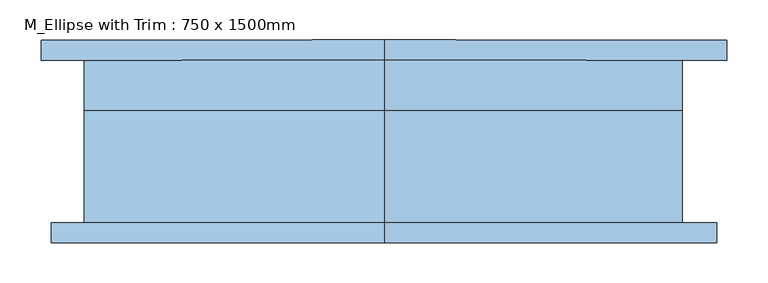
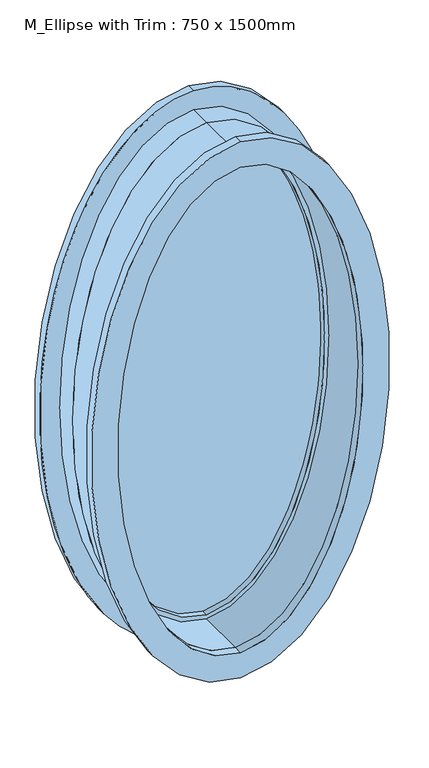
"""IFC4 building model written with IfcOpenShell, lengths in millimetres: window geometry, M_Ellipse with Trim : 750 x 1500mm."""

from ifc_helpers import new_model, si_unit, point, frame, origin, place, context, project, spatial, ellipse_curve, trimmed, source, transform, mapped, element, save
from ifc_brep_helpers import plane_surface, extruded_surface, advanced_brep


def m_ellipse_with_trim_750_x_1500mm_90dfdbfc(model_context):
    return source(origin(), model_context, "Body", "AdvancedBrep", [
        advanced_brep(
        [(0.0, -101.6, 2415.0), (0.0, -101.6, 915.0), (0.0, -101.6, 2383.25), (0.0, -101.6, 946.75), (0.0, 38.1, 2415.0), (0.0, 38.1, 915.0), (0.0, 38.1, 2383.25), (0.0, 38.1, 946.75)],
        [
            (0, 1, ellipse_curve(frame((0.0, -101.6, 1665.0), z_axis=(0.0, -1.0, 0.0), x_axis=(0.0, 0.0, -1.0)), 750.0, 375.0)),
            (1, 0, ellipse_curve(frame((0.0, -101.6, 1665.0), z_axis=(0.0, -1.0, 0.0), x_axis=(0.0, 0.0, -1.0)), 750.0, 375.0)),
            (2, 3, ellipse_curve(frame((0.0, -101.6, 1665.0), z_axis=(0.0, 1.0, 0.0), x_axis=(0.0, 0.0, -1.0)), 718.25, 343.25)),
            (3, 2, ellipse_curve(frame((0.0, -101.6, 1665.0), z_axis=(0.0, 1.0, 0.0), x_axis=(0.0, 0.0, -1.0)), 718.25, 343.25)),
            (0, 4),
            (4, 5, ellipse_curve(frame((0.0, 38.1, 1665.0), z_axis=(0.0, -1.0, 0.0), x_axis=(0.0, 0.0, -1.0)), 750.0, 375.0)),
            (5, 1),
            (5, 4, ellipse_curve(frame((0.0, 38.1, 1665.0), z_axis=(0.0, -1.0, 0.0), x_axis=(0.0, 0.0, -1.0)), 750.0, 375.0)),
            (2, 6),
            (6, 7, ellipse_curve(frame((0.0, 38.1, 1665.0), z_axis=(0.0, 1.0, 0.0), x_axis=(0.0, 0.0, -1.0)), 718.25, 343.25)),
            (7, 3),
            (7, 6, ellipse_curve(frame((0.0, 38.1, 1665.0), z_axis=(0.0, 1.0, 0.0), x_axis=(0.0, 0.0, -1.0)), 718.25, 343.25)),
        ],
        [
            plane_surface(frame((0.0, -101.6, 915.0), z_axis=(0.0, -1.0, 0.0), x_axis=(1.0, 0.0, 0.0))),
            extruded_surface(trimmed(ellipse_curve(frame((0.0, 177.8, 1665.0), z_axis=(0.0, -1.0, 0.0), x_axis=(0.0, 0.0, -1.0)), 750.0, 375.0), [point((0.0, 177.8, 2415.0))], [point((0.0, 177.8, 915.0))], True, "CARTESIAN"), (0.0, -139.70000000000002, 0.0), 139.70000000000002),
            extruded_surface(trimmed(ellipse_curve(frame((0.0, 177.8, 1665.0), z_axis=(0.0, -1.0, 0.0), x_axis=(0.0, 0.0, -1.0)), 750.0, 375.0), [point((0.0, 177.8, 915.0))], [point((0.0, 177.8, 2415.0))], True, "CARTESIAN"), (0.0, -139.70000000000002, 0.0), 139.70000000000002),
            extruded_surface(trimmed(ellipse_curve(frame((0.0, 38.1, 1665.0), z_axis=(0.0, 1.0, 0.0), x_axis=(0.0, 0.0, -1.0)), 718.25, 343.25), [point((0.0, 38.1, 2383.25))], [point((0.0, 38.1, 946.75))], True, "CARTESIAN"), (0.0, -139.7, 0.0), 139.7),
            extruded_surface(trimmed(ellipse_curve(frame((0.0, 38.1, 1665.0), z_axis=(0.0, 1.0, 0.0), x_axis=(0.0, 0.0, -1.0)), 718.25, 343.25), [point((0.0, 38.1, 946.75))], [point((0.0, 38.1, 2383.25))], True, "CARTESIAN"), (0.0, -139.7, 0.0), 139.7),
            plane_surface(frame((0.0, 38.1, 915.0), z_axis=(0.0, 1.0, 0.0), x_axis=(-1.0, 0.0, 0.0))),
        ],
        [
            (0, [[1, 2], [3, 4]]),
            (1, [[-1, 5, 6, 7]]),
            (2, [[-2, -7, 8, -5]]),
            (3, [[-3, 9, 10, 11]]),
            (4, [[-4, -11, 12, -9]]),
            (5, [[-8, -6], [-12, -10]]),
        ],
    ),
        advanced_brep(
        [(0.0, 55.3459129, 2370.55), (0.0, 55.3459129, 959.45), (0.0, 64.8706843, 2370.55), (0.0, 64.8706843, 959.45)],
        [
            (0, 1, ellipse_curve(frame((0.0, 55.3459129, 1665.0), z_axis=(0.0, -1.0, 0.0), x_axis=(0.0, 0.0, -1.0)), 705.55, 330.55)),
            (1, 0, ellipse_curve(frame((0.0, 55.3459129, 1665.0), z_axis=(0.0, -1.0, 0.0), x_axis=(0.0, 0.0, -1.0)), 705.55, 330.55)),
            (0, 2),
            (2, 3, ellipse_curve(frame((0.0, 64.8706843, 1665.0), z_axis=(0.0, -1.0, 0.0), x_axis=(0.0, 0.0, -1.0)), 705.55, 330.55)),
            (3, 1),
            (3, 2, ellipse_curve(frame((0.0, 64.8706843, 1665.0), z_axis=(0.0, -1.0, 0.0), x_axis=(0.0, 0.0, -1.0)), 705.55, 330.55)),
        ],
        [
            plane_surface(frame((0.0, 55.3459129, 959.45), z_axis=(0.0, -1.0, 0.0), x_axis=(1.0, 0.0, 0.0))),
            extruded_surface(trimmed(ellipse_curve(frame((0.0, 74.3954558, 1665.0), z_axis=(0.0, -1.0, 0.0), x_axis=(0.0, 0.0, -1.0)), 705.55, 330.55), [point((0.0, 74.3954558, 2370.55))], [point((0.0, 74.3954558, 959.45))], True, "CARTESIAN"), (0.0, -9.5247715, 0.0), 9.5247715),
            extruded_surface(trimmed(ellipse_curve(frame((0.0, 74.3954558, 1665.0), z_axis=(0.0, -1.0, 0.0), x_axis=(0.0, 0.0, -1.0)), 705.55, 330.55), [point((0.0, 74.3954558, 959.45))], [point((0.0, 74.3954558, 2370.55))], True, "CARTESIAN"), (0.0, -9.5247715, 0.0), 9.5247715),
            plane_surface(frame((0.0, 64.8706843, 959.45), z_axis=(0.0, 1.0, 0.0), x_axis=(-1.0, 0.0, 0.0))),
        ],
        [
            (0, [[1, 2]]),
            (1, [[-1, 3, 4, 5]]),
            (2, [[-2, -5, 6, -3]]),
            (3, [[-6, -4]]),
        ],
    ),
        advanced_brep(
        [(0.0, 38.1, 2395.95), (0.0, 38.1, 934.05), (0.0, 38.1, 2370.55), (0.0, 38.1, 959.45), (0.0, 82.55, 2395.95), (0.0, 82.55, 934.05), (0.0, 82.55, 2370.55), (0.0, 82.55, 959.45)],
        [
            (0, 1, ellipse_curve(frame((0.0, 38.1, 1665.0), z_axis=(0.0, -1.0, 0.0), x_axis=(0.0, 0.0, -1.0)), 730.95, 355.95)),
            (1, 0, ellipse_curve(frame((0.0, 38.1, 1665.0), z_axis=(0.0, -1.0, 0.0), x_axis=(0.0, 0.0, -1.0)), 730.95, 355.95)),
            (2, 3, ellipse_curve(frame((0.0, 38.1, 1665.0), z_axis=(0.0, 1.0, 0.0), x_axis=(0.0, 0.0, -1.0)), 705.55, 330.55)),
            (3, 2, ellipse_curve(frame((0.0, 38.1, 1665.0), z_axis=(0.0, 1.0, 0.0), x_axis=(0.0, 0.0, -1.0)), 705.55, 330.55)),
            (0, 4),
            (4, 5, ellipse_curve(frame((0.0, 82.55, 1665.0), z_axis=(0.0, -1.0, 0.0), x_axis=(0.0, 0.0, -1.0)), 730.95, 355.95)),
            (5, 1),
            (5, 4, ellipse_curve(frame((0.0, 82.55, 1665.0), z_axis=(0.0, -1.0, 0.0), x_axis=(0.0, 0.0, -1.0)), 730.95, 355.95)),
            (2, 6),
            (6, 7, ellipse_curve(frame((0.0, 82.55, 1665.0), z_axis=(0.0, 1.0, 0.0), x_axis=(0.0, 0.0, -1.0)), 705.55, 330.55)),
            (7, 3),
            (7, 6, ellipse_curve(frame((0.0, 82.55, 1665.0), z_axis=(0.0, 1.0, 0.0), x_axis=(0.0, 0.0, -1.0)), 705.55, 330.55)),
        ],
        [
            plane_surface(frame((0.0, 38.1, 934.05), z_axis=(0.0, -1.0, 0.0), x_axis=(1.0, 0.0, 0.0))),
            extruded_surface(trimmed(ellipse_curve(frame((0.0, 127.0, 1665.0), z_axis=(0.0, -1.0, 0.0), x_axis=(0.0, 0.0, -1.0)), 730.95, 355.95), [point((0.0, 127.0, 2395.95))], [point((0.0, 127.0, 934.05))], True, "CARTESIAN"), (0.0, -44.45, 0.0), 44.45),
            extruded_surface(trimmed(ellipse_curve(frame((0.0, 127.0, 1665.0), z_axis=(0.0, -1.0, 0.0), x_axis=(0.0, 0.0, -1.0)), 730.95, 355.95), [point((0.0, 127.0, 934.05))], [point((0.0, 127.0, 2395.95))], True, "CARTESIAN"), (0.0, -44.45, 0.0), 44.45),
            extruded_surface(trimmed(ellipse_curve(frame((0.0, 146.05, 1665.0), z_axis=(0.0, 1.0, 0.0), x_axis=(0.0, 0.0, -1.0)), 705.55, 330.55), [point((0.0, 146.05, 2370.55))], [point((0.0, 146.05, 959.45))], True, "CARTESIAN"), (0.0, -44.45000000000002, 0.0), 44.45000000000002),
            extruded_surface(trimmed(ellipse_curve(frame((0.0, 146.05, 1665.0), z_axis=(0.0, 1.0, 0.0), x_axis=(0.0, 0.0, -1.0)), 705.55, 330.55), [point((0.0, 146.05, 959.45))], [point((0.0, 146.05, 2370.55))], True, "CARTESIAN"), (0.0, -44.45000000000002, 0.0), 44.45000000000002),
            plane_surface(frame((0.0, 82.55, 934.05), z_axis=(0.0, 1.0, 0.0), x_axis=(-1.0, 0.0, 0.0))),
        ],
        [
            (0, [[1, 2], [3, 4]]),
            (1, [[-1, 5, 6, 7]]),
            (2, [[-2, -7, 8, -5]]),
            (3, [[-3, 9, 10, 11]]),
            (4, [[-4, -11, 12, -9]]),
            (5, [[-8, -6], [-12, -10]]),
        ],
    ),
        advanced_brep(
        [(0.0, 38.1, 2415.0), (0.0, 38.1, 915.0), (0.0, 38.1, 2395.95), (0.0, 38.1, 934.05), (0.0, 101.6, 2415.0), (0.0, 101.6, 915.0), (0.0, 101.6, 2395.95), (0.0, 101.6, 934.05)],
        [
            (0, 1, ellipse_curve(frame((0.0, 38.1, 1665.0), z_axis=(0.0, -1.0, 0.0), x_axis=(0.0, 0.0, -1.0)), 750.0, 375.0)),
            (1, 0, ellipse_curve(frame((0.0, 38.1, 1665.0), z_axis=(0.0, -1.0, 0.0), x_axis=(0.0, 0.0, -1.0)), 750.0, 375.0)),
            (2, 3, ellipse_curve(frame((0.0, 38.1, 1665.0), z_axis=(0.0, 1.0, 0.0), x_axis=(0.0, 0.0, -1.0)), 730.95, 355.95)),
            (3, 2, ellipse_curve(frame((0.0, 38.1, 1665.0), z_axis=(0.0, 1.0, 0.0), x_axis=(0.0, 0.0, -1.0)), 730.95, 355.95)),
            (0, 4),
            (4, 5, ellipse_curve(frame((0.0, 101.6, 1665.0), z_axis=(0.0, -1.0, 0.0), x_axis=(0.0, 0.0, -1.0)), 750.0, 375.0)),
            (5, 1),
            (5, 4, ellipse_curve(frame((0.0, 101.6, 1665.0), z_axis=(0.0, -1.0, 0.0), x_axis=(0.0, 0.0, -1.0)), 750.0, 375.0)),
            (2, 6),
            (6, 7, ellipse_curve(frame((0.0, 101.6, 1665.0), z_axis=(0.0, 1.0, 0.0), x_axis=(0.0, 0.0, -1.0)), 730.95, 355.95)),
            (7, 3),
            (7, 6, ellipse_curve(frame((0.0, 101.6, 1665.0), z_axis=(0.0, 1.0, 0.0), x_axis=(0.0, 0.0, -1.0)), 730.95, 355.95)),
        ],
        [
            plane_surface(frame((0.0, 38.1, 915.0), z_axis=(0.0, -1.0, 0.0), x_axis=(1.0, 0.0, 0.0))),
            extruded_surface(trimmed(ellipse_curve(frame((0.0, 165.1, 1665.0), z_axis=(0.0, -1.0, 0.0), x_axis=(0.0, 0.0, -1.0)), 750.0, 375.0), [point((0.0, 165.1, 2415.0))], [point((0.0, 165.1, 915.0))], True, "CARTESIAN"), (0.0, -63.5, 0.0), 63.5),
            extruded_surface(trimmed(ellipse_curve(frame((0.0, 165.1, 1665.0), z_axis=(0.0, -1.0, 0.0), x_axis=(0.0, 0.0, -1.0)), 750.0, 375.0), [point((0.0, 165.1, 915.0))], [point((0.0, 165.1, 2415.0))], True, "CARTESIAN"), (0.0, -63.5, 0.0), 63.5),
            extruded_surface(trimmed(ellipse_curve(frame((0.0, 165.1, 1665.0), z_axis=(0.0, 1.0, 0.0), x_axis=(0.0, 0.0, -1.0)), 730.95, 355.95), [point((0.0, 165.1, 2395.95))], [point((0.0, 165.1, 934.05))], True, "CARTESIAN"), (0.0, -63.5, 0.0), 63.5),
            extruded_surface(trimmed(ellipse_curve(frame((0.0, 165.1, 1665.0), z_axis=(0.0, 1.0, 0.0), x_axis=(0.0, 0.0, -1.0)), 730.95, 355.95), [point((0.0, 165.1, 934.05))], [point((0.0, 165.1, 2395.95))], True, "CARTESIAN"), (0.0, -63.5, 0.0), 63.5),
            plane_surface(frame((0.0, 101.6, 915.0), z_axis=(0.0, 1.0, 0.0), x_axis=(-1.0, 0.0, 0.0))),
        ],
        [
            (0, [[1, 2], [3, 4]]),
            (1, [[-1, 5, 6, 7]]),
            (2, [[-2, -7, 8, -5]]),
            (3, [[-3, 9, 10, 11]]),
            (4, [[-4, -11, 12, -9]]),
            (5, [[-8, -6], [-12, -10]]),
        ],
    ),
        advanced_brep(
        [(0.0, -126.6, 2458.25), (0.0, -126.6, 871.75), (0.0, -126.6, 2383.25), (0.0, -126.6, 946.75), (0.0, -101.6, 2458.25), (0.0, -101.6, 871.75), (0.0, -101.6, 2383.25), (0.0, -101.6, 946.75)],
        [
            (0, 1, ellipse_curve(frame((0.0, -126.6, 1665.0), z_axis=(0.0, -1.0, 0.0), x_axis=(0.0, 0.0, -1.0)), 793.25, 418.25)),
            (1, 0, ellipse_curve(frame((0.0, -126.6, 1665.0), z_axis=(0.0, -1.0, 0.0), x_axis=(0.0, 0.0, -1.0)), 793.25, 418.25)),
            (2, 3, ellipse_curve(frame((0.0, -126.6, 1665.0), z_axis=(0.0, 1.0, 0.0), x_axis=(0.0, 0.0, -1.0)), 718.25, 343.25)),
            (3, 2, ellipse_curve(frame((0.0, -126.6, 1665.0), z_axis=(0.0, 1.0, 0.0), x_axis=(0.0, 0.0, -1.0)), 718.25, 343.25)),
            (4, 5, ellipse_curve(frame((0.0, -101.6, 1665.0), z_axis=(0.0, 1.0, 0.0), x_axis=(0.0, 0.0, -1.0)), 793.25, 418.25)),
            (5, 4, ellipse_curve(frame((0.0, -101.6, 1665.0), z_axis=(0.0, 1.0, 0.0), x_axis=(0.0, 0.0, -1.0)), 793.25, 418.25)),
            (6, 7, ellipse_curve(frame((0.0, -101.6, 1665.0), z_axis=(0.0, -1.0, 0.0), x_axis=(0.0, 0.0, -1.0)), 718.25, 343.25)),
            (7, 6, ellipse_curve(frame((0.0, -101.6, 1665.0), z_axis=(0.0, -1.0, 0.0), x_axis=(0.0, 0.0, -1.0)), 718.25, 343.25)),
            (2, 6),
            (7, 3),
            (0, 4),
            (5, 1),
        ],
        [
            plane_surface(frame((0.0, -126.6, 946.75), z_axis=(0.0, -1.0, 0.0), x_axis=(-1.0, 0.0, 0.0))),
            plane_surface(frame((0.0, -101.6, 946.75), z_axis=(0.0, 1.0, 0.0), x_axis=(1.0, 0.0, 0.0))),
            extruded_surface(trimmed(ellipse_curve(frame((0.0, -76.6, 1665.0), z_axis=(0.0, 1.0, 0.0), x_axis=(0.0, 0.0, -1.0)), 718.25, 343.25), [point((0.0, -76.6, 2383.25))], [point((0.0, -76.6, 946.75))], True, "CARTESIAN"), (0.0, -25.0, 0.0), 25.0),
            extruded_surface(trimmed(ellipse_curve(frame((0.0, -76.6, 1665.0), z_axis=(0.0, 1.0, 0.0), x_axis=(0.0, 0.0, -1.0)), 718.25, 343.25), [point((0.0, -76.6, 946.75))], [point((0.0, -76.6, 2383.25))], True, "CARTESIAN"), (0.0, -25.0, 0.0), 25.0),
            extruded_surface(trimmed(ellipse_curve(frame((0.0, -76.6, 1665.0), z_axis=(0.0, -1.0, 0.0), x_axis=(0.0, 0.0, -1.0)), 793.25, 418.25), [point((0.0, -76.6, 2458.25))], [point((0.0, -76.6, 871.75))], True, "CARTESIAN"), (0.0, -25.0, 0.0), 25.0),
            extruded_surface(trimmed(ellipse_curve(frame((0.0, -76.6, 1665.0), z_axis=(0.0, -1.0, 0.0), x_axis=(0.0, 0.0, -1.0)), 793.25, 418.25), [point((0.0, -76.6, 871.75))], [point((0.0, -76.6, 2458.25))], True, "CARTESIAN"), (0.0, -25.0, 0.0), 25.0),
        ],
        [
            (0, [[1, 2], [3, 4]]),
            (1, [[5, 6], [7, 8]]),
            (2, [[-3, 9, -8, 10]]),
            (3, [[-4, -10, -7, -9]]),
            (4, [[-1, 11, -6, 12]]),
            (5, [[-2, -12, -5, -11]]),
        ],
    ),
        advanced_brep(
        [(0.0, 101.6, 2470.95), (0.0, 101.6, 859.05), (0.0, 101.6, 2395.95), (0.0, 101.6, 934.05), (0.0, 126.6, 2470.95), (0.0, 126.6, 859.05), (0.0, 126.6, 2395.95), (0.0, 126.6, 934.05)],
        [
            (0, 1, ellipse_curve(frame((0.0, 101.6, 1665.0), z_axis=(0.0, -1.0, 0.0), x_axis=(0.0, 0.0, -1.0)), 805.95, 430.95)),
            (1, 0, ellipse_curve(frame((0.0, 101.6, 1665.0), z_axis=(0.0, -1.0, 0.0), x_axis=(0.0, 0.0, -1.0)), 805.95, 430.95)),
            (2, 3, ellipse_curve(frame((0.0, 101.6, 1665.0), z_axis=(0.0, 1.0, 0.0), x_axis=(0.0, 0.0, -1.0)), 730.95, 355.95)),
            (3, 2, ellipse_curve(frame((0.0, 101.6, 1665.0), z_axis=(0.0, 1.0, 0.0), x_axis=(0.0, 0.0, -1.0)), 730.95, 355.95)),
            (4, 5, ellipse_curve(frame((0.0, 126.6, 1665.0), z_axis=(0.0, 1.0, 0.0), x_axis=(0.0, 0.0, -1.0)), 805.95, 430.95)),
            (5, 4, ellipse_curve(frame((0.0, 126.6, 1665.0), z_axis=(0.0, 1.0, 0.0), x_axis=(0.0, 0.0, -1.0)), 805.95, 430.95)),
            (6, 7, ellipse_curve(frame((0.0, 126.6, 1665.0), z_axis=(0.0, -1.0, 0.0), x_axis=(0.0, 0.0, -1.0)), 730.95, 355.95)),
            (7, 6, ellipse_curve(frame((0.0, 126.6, 1665.0), z_axis=(0.0, -1.0, 0.0), x_axis=(0.0, 0.0, -1.0)), 730.95, 355.95)),
            (2, 6),
            (7, 3),
            (0, 4),
            (5, 1),
        ],
        [
            plane_surface(frame((0.0, 101.6, 934.05), z_axis=(0.0, -1.0, 0.0), x_axis=(-1.0, 0.0, 0.0))),
            plane_surface(frame((0.0, 126.6, 934.05), z_axis=(0.0, 1.0, 0.0), x_axis=(1.0, 0.0, 0.0))),
            extruded_surface(trimmed(ellipse_curve(frame((0.0, 151.6, 1665.0), z_axis=(0.0, 1.0, 0.0), x_axis=(0.0, 0.0, -1.0)), 730.95, 355.95), [point((0.0, 151.6, 2395.95))], [point((0.0, 151.6, 934.05))], True, "CARTESIAN"), (0.0, -25.0, 0.0), 25.0),
            extruded_surface(trimmed(ellipse_curve(frame((0.0, 151.6, 1665.0), z_axis=(0.0, 1.0, 0.0), x_axis=(0.0, 0.0, -1.0)), 730.95, 355.95), [point((0.0, 151.6, 934.05))], [point((0.0, 151.6, 2395.95))], True, "CARTESIAN"), (0.0, -25.0, 0.0), 25.0),
            extruded_surface(trimmed(ellipse_curve(frame((0.0, 126.6, 1665.0), z_axis=(0.0, -1.0, 0.0), x_axis=(0.0, 0.0, -1.0)), 805.95, 430.95), [point((0.0, 126.6, 2470.95))], [point((0.0, 126.6, 859.05))], True, "CARTESIAN"), (0.0, -25.0, 0.0), 25.0),
            extruded_surface(trimmed(ellipse_curve(frame((0.0, 126.6, 1665.0), z_axis=(0.0, -1.0, 0.0), x_axis=(0.0, 0.0, -1.0)), 805.95, 430.95), [point((0.0, 126.6, 859.05))], [point((0.0, 126.6, 2470.95))], True, "CARTESIAN"), (0.0, -25.0, 0.0), 25.0),
        ],
        [
            (0, [[1, 2], [3, 4]]),
            (1, [[5, 6], [7, 8]]),
            (2, [[-3, 9, -8, 10]]),
            (3, [[-4, -10, -7, -9]]),
            (4, [[-1, 11, -6, 12]]),
            (5, [[-2, -12, -5, -11]]),
        ],
    ),
    ])


if __name__ == "__main__":
    model = new_model("IFC4")
    model_context = context("Model", 3, world=origin())
    ifc_project = project(units=[si_unit("LENGTHUNIT", "METRE", prefix="MILLI")], contexts=[model_context])
    site = spatial("IfcSite", under=ifc_project)
    building = spatial("IfcBuilding", under=site)
    placement = place(None, origin())
    m_ellipse_with_trim_750_x_1500mm_shape = m_ellipse_with_trim_750_x_1500mm_90dfdbfc(model_context)
    element("IfcWindow", 1, ObjectType="M_Ellipse with Trim : 750 x 1500mm", at=placement, inside=building, context=model_context, shape_type="MappedRepresentation", body=[
        mapped(m_ellipse_with_trim_750_x_1500mm_shape, transform((0.0, 0.0, 0.0), x_axis=(1.0, 0.0, 0.0), y_axis=(0.0, 1.0, 0.0), z_axis=(0.0, 0.0, 1.0))),
    ])
    save(model, "model.ifc")

# Revit data of these elements
# Type "M_Ellipse with Trim : 750 x 1500mm"
#   Type Mark = "20"
#   Construction Type Id = "GSP4R"
#   Analytic Construction = "1/8 in Pilkington single glazing"
#   Visual Light Transmittance = 0.9
#   Thermal Resistance (R) = 0.1491 (m²·K)/W
#   Solar Heat Gain Coefficient = 0.86
#   Height = 4' - 11.05512"
#   Heat Transfer Coefficient (U) = 6.7069 W/(m²·K)
#   Half Width = 1' - 2.76378"
#   Half Height = 2' - 5.52756"
#   Default Sill Height = 3' - 0.02362"
#   Trim Projection = 0' - 0.98425"
#   Trim Width = 0' - 2.95276"
#   Width = 2' - 5.52756"
#   Trim Material = none
#   Sash Material = none
#   Wall Closure = (empty or 0)
# Element 1 (IfcWindow, "M_Ellipse with Trim : 750 x 1500mm")
#   Materials on its faces: "Glass"
# Materials
#   "Glass": class "Glass", colour RGB 0 128 192, transparency 0.75, Description = "Soda Lime Glass", Cost = 0
